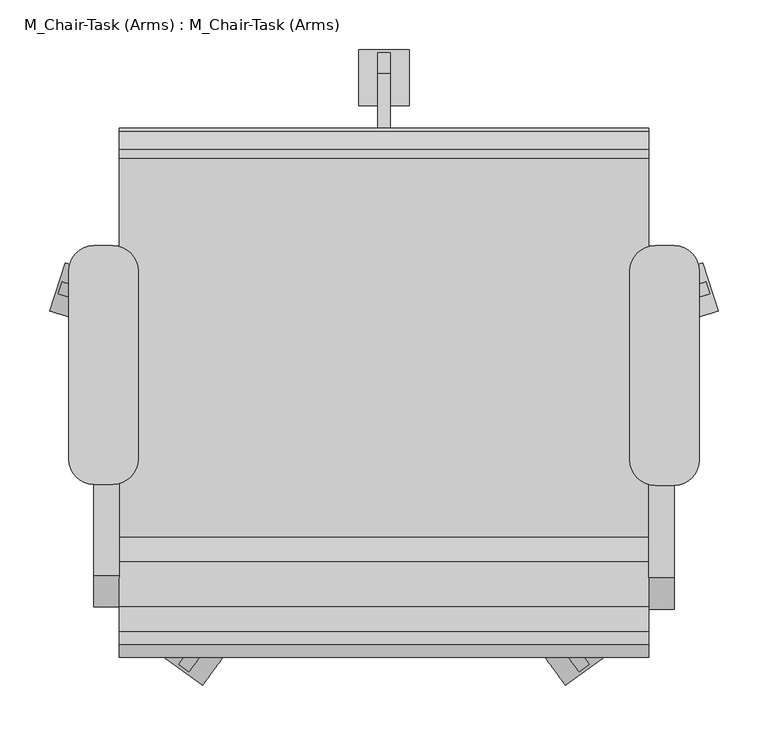
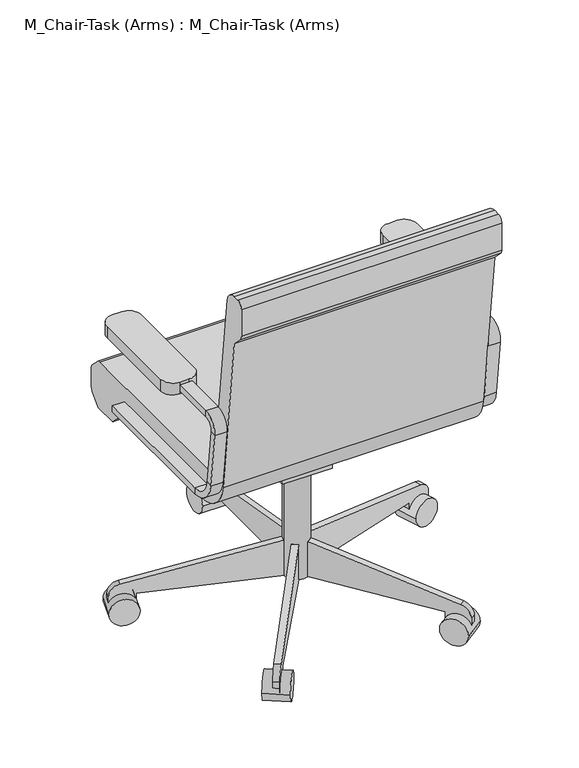
"""IFC4 building model written with IfcOpenShell, lengths in millimetres: furniture geometry, M_Chair-Task (Arms) : M_Chair-Task (Arms)."""

from ifc_helpers import new_model, si_unit, point, frame, frame_2d, origin, place, context, project, spatial, polyline, circle_curve, trimmed, segment, composite_curve, outline, extrude, source, transform, mapped, element, save
from ifc_brep_helpers import plane_surface, cylinder_surface, revolved_surface, advanced_brep


def m_chair_task_arms_m_chair_task_arms_bb362225(model_context):
    return source(origin(), model_context, "Body", "SolidModel", [
        extrude(outline(composite_curve([segment(polyline([(-126.2050455, 457.2), (255.0102301, 457.2)]), True, "CONTINUOUS"), segment(trimmed(circle_curve(frame_2d((255.0102301, 444.5)), 12.7), [point((255.0102301, 457.2))], [point((263.9604301, 453.510212))], False, "CARTESIAN"), True, "CONTINUOUS"), segment(polyline([(263.9604301, 453.510212), (281.8961016, 435.6939999)]), True, "CONTINUOUS"), segment(trimmed(circle_curve(frame_2d((272.9459016, 426.6837879)), 12.7), [point((281.8961016, 435.6939999))], [point((285.6459016, 426.6837879))], False, "CARTESIAN"), True, "CONTINUOUS"), segment(polyline([(285.6459016, 426.6837879), (285.6459016, 391.6405184)]), True, "CONTINUOUS"), segment(trimmed(circle_curve(frame_2d((260.2459016, 391.6405184)), 25.4), [point((285.6459016, 391.6405184))], [point((278.2663256, 373.7401184))], False, "CARTESIAN"), True, "CONTINUOUS"), segment(polyline([(278.2663256, 373.7401184), (260.2470284, 355.6), (209.4470284, 355.6), (181.0744602, 383.7835944), (-107.1089978, 383.7835944)]), True, "CONTINUOUS"), segment(trimmed(circle_curve(frame_2d((-107.1089978, 459.9835944)), 76.2), [point((-107.1089978, 383.7835944))], [point((-182.7870738, 451.0802913))], False, "CARTESIAN"), True, "CONTINUOUS"), segment(polyline([(-182.7870738, 451.0802913), (-222.3540984, 787.4), (-244.0343545, 809.0802561)]), True, "CONTINUOUS"), segment(trimmed(circle_curve(frame_2d((-235.0540984, 818.0605122)), 12.7), [point((-244.0343545, 809.0802561))], [point((-247.7540984, 818.0605122))], False, "CARTESIAN"), True, "CONTINUOUS"), segment(polyline([(-247.7540984, 818.0605122), (-247.7540984, 876.3)]), True, "CONTINUOUS"), segment(trimmed(circle_curve(frame_2d((-235.0540984, 876.3)), 12.7), [point((-247.7540984, 876.3))], [point((-235.0540984, 889.0))], False, "CARTESIAN"), True, "CONTINUOUS"), segment(polyline([(-235.0540984, 889.0), (-222.1789239, 889.0)]), True, "CONTINUOUS"), segment(trimmed(circle_curve(frame_2d((-222.1789239, 863.6)), 25.4), [point((-222.1789239, 889.0))], [point((-196.9528985, 866.5677677))], False, "CARTESIAN"), True, "CONTINUOUS"), segment(polyline([(-196.9528985, 866.5677677), (-151.4310708, 479.6322323)]), True, "CONTINUOUS"), segment(trimmed(circle_curve(frame_2d((-126.2050455, 482.6)), 25.4), [point((-151.4310708, 479.6322323))], [point((-126.2050455, 457.2))], True, "CARTESIAN"), True, "CONTINUOUS")], self_intersect=False)), frame((-125.7091803, 0.0, 0.0), z_axis=(1.0, 0.0, 0.0), x_axis=(0.0, 1.0, 0.0)), (0.0, 0.0, 1.0), 533.4),
        extrude(outline(polyline([(69.7459016, 383.7835944), (69.7459016, 371.0835944), (18.9459016, 283.0954134), (-19.1540984, 283.0954134), (-19.1540984, 383.7835944), (69.7459016, 383.7835944)])), frame((90.1908197, 0.0, 0.0), z_axis=(1.0, 0.0, 0.0), x_axis=(0.0, 1.0, 0.0)), (0.0, 0.0, 1.0), 101.6),
        extrude(outline(composite_curve([segment(polyline([(311.0459016, 53.5835944), (18.9459016, 53.5835944), (18.9459016, 129.7835944), (44.3459016, 129.7835944), (340.8565654, 77.5007643)]), True, "CONTINUOUS"), segment(trimmed(circle_curve(frame_2d((336.4459016, 52.4866474)), 25.4), [point((340.8565654, 77.5007643))], [point((361.8459016, 52.4866474))], False, "CARTESIAN"), True, "CONTINUOUS"), segment(polyline([(361.8459016, 52.4866474), (361.8459016, 28.1835944), (311.0459016, 28.1835944), (311.0459016, 53.5835944)]), True, "CONTINUOUS")], self_intersect=False)), frame((134.6408197, 0.0, 0.0), z_axis=(1.0, 0.0, 0.0), x_axis=(0.0, 1.0, 0.0)), (0.0, 0.0, 1.0), 12.7),
        extrude(outline(composite_curve([segment(trimmed(circle_curve(frame_2d((336.4459016, 28.1835944)), 28.2002727), [point((308.2456289, 28.1835944))], [point((364.6461744, 28.1835944))], False, "CARTESIAN"), True, "CONTINUOUS"), segment(trimmed(circle_curve(frame_2d((336.4459016, 28.1835944)), 28.2002727), [point((364.6461744, 28.1835944))], [point((308.2456289, 28.1835944))], False, "CARTESIAN"), True, "CONTINUOUS")], self_intersect=False)), frame((115.5908197, 0.0, 0.0), z_axis=(1.0, 0.0, 0.0), x_axis=(0.0, 1.0, 0.0)), (0.0, 0.0, 1.0), 50.8),
        extrude(outline(composite_curve([segment(polyline([(25.4, 0.0), (25.4, 292.1000001), (101.6, 292.1000001), (101.6, 266.7), (49.3171699, -29.8106636)]), True, "CONTINUOUS"), segment(trimmed(circle_curve(frame_2d((24.303053, -25.4)), 25.4), [point((49.3171699, -29.8106636))], [point((24.303053, -50.8))], False, "CARTESIAN"), True, "CONTINUOUS"), segment(polyline([(24.303053, -50.8), (0.0, -50.8), (0.0, 0.0), (25.4, 0.0)]), True, "CONTINUOUS")], self_intersect=False)), frame((-138.7750467, 103.1705568, 28.1835944), z_axis=(0.3090169943749487, 0.9510565162951532, 0.0), x_axis=(0.0, 0.0, 1.0)), (0.0, 0.0, 1.0), 12.7),
        extrude(outline(composite_curve([segment(trimmed(circle_curve(frame_2d((0.0, -28.2002727)), 28.2002727), [point((0.0, -56.4005454))], [point((0.0, 0.0))], False, "CARTESIAN"), True, "CONTINUOUS"), segment(trimmed(circle_curve(frame_2d((0.0, -28.2002727)), 28.2002727), [point((0.0, 0.0))], [point((0.0, -56.4005454))], False, "CARTESIAN"), True, "CONTINUOUS")], self_intersect=False)), frame((-195.638709, 101.6163254, 28.1835944), z_axis=(0.3090169943749487, 0.9510565162951532, 0.0), x_axis=(0.0, 0.0, -1.0)), (0.0, 0.0, 1.0), 50.8),
        extrude(outline(composite_curve([segment(polyline([(25.4, 0.0), (25.4, 292.1), (101.6, 292.1), (101.6, 266.7), (49.3171699, -29.8106637)]), True, "CONTINUOUS"), segment(trimmed(circle_curve(frame_2d((24.303053, -25.3999999)), 25.4), [point((49.3171699, -29.8106637))], [point((24.303053, -50.8))], False, "CARTESIAN"), True, "CONTINUOUS"), segment(polyline([(24.303053, -50.8), (0.0, -50.8), (0.0, 0.0), (25.4, 0.0)]), True, "CONTINUOUS")], self_intersect=False)), frame((-25.5639946, -221.1003988, 28.1835944), z_axis=(-0.8090169943749459, 0.5877852522924754, 0.0), x_axis=(0.0, 0.0, 1.0)), (0.0, 0.0, 1.0), 12.7),
        extrude(outline(composite_curve([segment(trimmed(circle_curve(frame_2d((0.0, -28.2002727)), 28.2002727), [point((0.0, -56.4005455))], [point((0.0, 0.0))], False, "CARTESIAN"), True, "CONTINUOUS"), segment(trimmed(circle_curve(frame_2d((0.0, -28.2002727)), 28.2002727), [point((0.0, 0.0))], [point((0.0, -56.4005455))], False, "CARTESIAN"), True, "CONTINUOUS")], self_intersect=False)), frame((-41.6576707, -275.6612394, 28.1835944), z_axis=(-0.8090169943749458, 0.5877852522924754, 0.0), x_axis=(0.0, 0.0, -1.0)), (0.0, 0.0, 1.0), 50.8),
        extrude(outline(composite_curve([segment(polyline([(-25.4, 0.0), (0.0, 0.0), (0.0, -50.8), (-24.303053, -50.8)]), True, "CONTINUOUS"), segment(trimmed(circle_curve(frame_2d((-24.303053, -25.3999999)), 25.4), [point((-24.303053, -50.8))], [point((-49.3171699, -29.8106636))], False, "CARTESIAN"), True, "CONTINUOUS"), segment(polyline([(-49.3171699, -29.8106636), (-101.6, 266.7), (-101.6, 292.1), (-25.4, 292.1), (-25.4, 0.0)]), True, "CONTINUOUS")], self_intersect=False)), frame((307.545634, -221.1003988, 28.1835944), z_axis=(0.8090169943749499, 0.5877852522924699, 0.0), x_axis=(0.0, 0.0, -1.0)), (0.0, 0.0, 1.0), 12.7),
        extrude(outline(composite_curve([segment(trimmed(circle_curve(frame_2d((0.0, -28.2002727)), 28.2002727), [point((0.0, -56.4005455))], [point((0.0, 0.0))], False, "CARTESIAN"), True, "CONTINUOUS"), segment(trimmed(circle_curve(frame_2d((0.0, -28.2002727)), 28.2002727), [point((0.0, 0.0))], [point((0.0, -56.4005455))], False, "CARTESIAN"), True, "CONTINUOUS")], self_intersect=False)), frame((323.63931, -275.6612394, 28.1835944), z_axis=(0.8090169943749499, 0.5877852522924699, 0.0), x_axis=(0.0, 0.0, 1.0)), (0.0, 0.0, 1.0), 50.8),
        extrude(outline(composite_curve([segment(polyline([(-25.4, 0.0), (0.0, 0.0), (0.0, -50.8), (-24.303053, -50.8)]), True, "CONTINUOUS"), segment(trimmed(circle_curve(frame_2d((-24.303053, -25.4)), 25.4), [point((-24.303053, -50.8))], [point((-49.3171699, -29.8106637))], False, "CARTESIAN"), True, "CONTINUOUS"), segment(polyline([(-49.3171699, -29.8106637), (-101.6, 266.7), (-101.6, 292.1), (-25.4, 292.1), (-25.4, 0.0)]), True, "CONTINUOUS")], self_intersect=False)), frame((420.756686, 103.1705568, 28.1835944), z_axis=(-0.3090169943749423, 0.9510565162951553, 0.0), x_axis=(0.0, 0.0, -1.0)), (0.0, 0.0, 1.0), 12.7),
        extrude(outline(composite_curve([segment(trimmed(circle_curve(frame_2d((0.0, -28.2002727)), 28.2002727), [point((0.0, -56.4005455))], [point((0.0, 0.0))], False, "CARTESIAN"), True, "CONTINUOUS"), segment(trimmed(circle_curve(frame_2d((0.0, -28.2002727)), 28.2002727), [point((0.0, 0.0))], [point((0.0, -56.4005455))], False, "CARTESIAN"), True, "CONTINUOUS")], self_intersect=False)), frame((477.6203484, 101.6163254, 28.1835944), z_axis=(-0.3090169943749423, 0.9510565162951553, 0.0), x_axis=(0.0, 0.0, 1.0)), (0.0, 0.0, 1.0), 50.8),
        extrude(outline(composite_curve([segment(trimmed(circle_curve(frame_2d((140.9908197, 18.9459016)), 25.4), [point((115.5908197, 18.9459016))], [point((166.3908197, 18.9459016))], False, "CARTESIAN"), True, "CONTINUOUS"), segment(trimmed(circle_curve(frame_2d((140.9908197, 18.9459016)), 25.4), [point((166.3908197, 18.9459016))], [point((115.5908197, 18.9459016))], False, "CARTESIAN"), True, "CONTINUOUS")], self_intersect=False)), frame((0.0, 0.0, 53.5835944), z_axis=(0.0, 0.0, 1.0), x_axis=(1.0, 0.0, 0.0)), (0.0, 0.0, 1.0), 330.5914056),
        advanced_brep(
        [(433.0908197, 167.0319091, 425.45), (433.0908197, 167.0319091, 412.75), (407.6908197, 167.0319091, 412.75), (407.6908197, 167.0319091, 425.45), (433.0908197, -128.329278, 425.45), (433.0908197, -128.329278, 412.75), (407.6908197, -128.329278, 412.75), (407.6908197, -128.329278, 425.45), (433.0908197, -185.0878351, 463.2225227), (433.0908197, -172.4748224, 464.7064065), (407.6908197, -185.0878351, 463.2225227), (407.6908197, -172.4748224, 464.7064065), (433.0908197, -186.2710303, 581.9741742), (433.0908197, -198.884043, 580.4902904), (407.6908197, -198.884043, 580.4902904), (407.6908197, -186.2710303, 581.9741742), (433.0908197, -167.3515113, 615.95), (433.0908197, -167.3515113, 603.25), (407.6908197, -167.3515113, 615.95), (407.6908197, -167.3515113, 603.25), (433.0908197, 18.9459016, 603.25), (407.6908197, 18.9459016, 603.25), (407.6908197, 18.9459016, 615.95), (433.0908197, 18.9459016, 615.95)],
        [
            (0, 1),
            (1, 2),
            (2, 3),
            (3, 0),
            (0, 4),
            (4, 5),
            (5, 1),
            (5, 6),
            (6, 2),
            (6, 7),
            (7, 3),
            (7, 4),
            (8, 5, circle_curve(frame((433.0908197, -128.329278, 469.9), z_axis=(1.0, 0.0, 0.0), x_axis=(0.0, 0.0, -1.0)), 57.15)),
            (4, 9, circle_curve(frame((433.0908197, -128.329278, 469.9), z_axis=(-1.0, 0.0, 0.0), x_axis=(0.0, 0.0, -1.0)), 44.45)),
            (9, 8),
            (10, 6, circle_curve(frame((407.6908197, -128.329278, 469.9), z_axis=(1.0, 0.0, 0.0), x_axis=(0.0, 0.0, -1.0)), 57.15)),
            (8, 10),
            (11, 7, circle_curve(frame((407.6908197, -128.329278, 469.9), z_axis=(1.0, 0.0, 0.0), x_axis=(0.0, 0.0, -1.0)), 44.45)),
            (10, 11),
            (11, 9),
            (9, 12),
            (12, 13),
            (13, 8),
            (13, 14),
            (14, 10),
            (14, 15),
            (15, 11),
            (15, 12),
            (16, 13, circle_curve(frame((433.0908197, -167.3515113, 584.2), z_axis=(1.0, 0.0, 0.0), x_axis=(0.0, -0.9931506043228767, -0.1168412475673929)), 31.75)),
            (12, 17, circle_curve(frame((433.0908197, -167.3515113, 584.2), z_axis=(-1.0, 0.0, 0.0), x_axis=(0.0, -0.9931506043228767, -0.1168412475673929)), 19.05)),
            (17, 16),
            (18, 14, circle_curve(frame((407.6908197, -167.3515113, 584.2), z_axis=(1.0, 0.0, 0.0), x_axis=(0.0, -0.9931506043228767, -0.1168412475673929)), 31.75)),
            (16, 18),
            (19, 15, circle_curve(frame((407.6908197, -167.3515113, 584.2), z_axis=(1.0, 0.0, 0.0), x_axis=(0.0, -0.9931506043228767, -0.1168412475673929)), 19.05)),
            (18, 19),
            (19, 17),
            (20, 21),
            (21, 22),
            (22, 23),
            (23, 20),
            (17, 20),
            (23, 16),
            (22, 18),
            (21, 19),
        ],
        [
            plane_surface(frame((406.191788, 167.0319091, 419.1), z_axis=(0.0, 1.0, 0.0), x_axis=(0.0, 0.0, -1.0))),
            plane_surface(frame((433.0908197, 167.0319091, 425.45), z_axis=(1.0, 0.0, 0.0), x_axis=(0.0, -1.0, 0.0))),
            plane_surface(frame((433.0908197, 167.0319091, 412.75), z_axis=(0.0, 0.0, -1.0), x_axis=(0.0, -1.0, 0.0))),
            plane_surface(frame((407.6908197, 167.0319091, 412.75), z_axis=(-1.0, 0.0, 0.0), x_axis=(0.0, -1.0, 0.0))),
            plane_surface(frame((407.6908197, 167.0319091, 425.45), z_axis=(0.0, 0.0, 1.0), x_axis=(0.0, -1.0, 0.0))),
            plane_surface(frame((433.0908197, -128.329278, 469.9), z_axis=(1.0, 0.0, 0.0), x_axis=(0.0, 0.0, -1.0))),
            cylinder_surface(frame((420.3908197, -128.329278, 469.9), z_axis=(-1.0, 0.0, 0.0), x_axis=(0.0, 0.0, -1.0)), 57.15),
            plane_surface(frame((407.6908197, -128.329278, 469.9), z_axis=(-1.0, 0.0, 0.0), x_axis=(0.0, 0.0, -1.0))),
            revolved_surface(polyline([(407.6908197, -128.329278, 425.45), (433.0908197, -128.329278, 425.45)]), (420.3908197, -128.329278, 469.9), (-1.0, 0.0, 0.0)),
            plane_surface(frame((433.0908197, -172.4748224, 464.7064065), z_axis=(1.0, 0.0, 0.0), x_axis=(0.0, -0.11684124756738626, 0.9931506043228775))),
            plane_surface(frame((433.0908197, -185.0878351, 463.2225227), z_axis=(0.0, -0.9931506043228775, -0.11684124756738655), x_axis=(0.0, -0.11684124756738655, 0.9931506043228775))),
            plane_surface(frame((407.6908197, -185.0878351, 463.2225227), z_axis=(-1.0, 0.0, 0.0), x_axis=(0.0, -0.11684124756738626, 0.9931506043228775))),
            plane_surface(frame((407.6908197, -172.4748224, 464.7064065), z_axis=(0.0, 0.9931506043228775, 0.11684124756738626), x_axis=(0.0, -0.11684124756738626, 0.9931506043228775))),
            plane_surface(frame((433.0908197, -167.3515113, 584.2), z_axis=(1.0, 0.0, 0.0), x_axis=(0.0, -0.9931506043228767, -0.1168412475673929))),
            cylinder_surface(frame((420.3908197, -167.3515113, 584.2), z_axis=(-1.0, 0.0, 0.0), x_axis=(0.0, -0.9931506043228767, -0.1168412475673929)), 31.75),
            plane_surface(frame((407.6908197, -167.3515113, 584.2), z_axis=(-1.0, 0.0, 0.0), x_axis=(0.0, -0.9931506043228767, -0.1168412475673929))),
            revolved_surface(polyline([(407.6908197, -186.2710303123508, 581.9741742338412), (433.0908197, -186.2710303123508, 581.9741742338412)]), (420.3908197, -167.3515113, 584.2), (-1.0, 0.0, 0.0)),
            plane_surface(frame((406.191788, 18.9459016, 609.6), z_axis=(0.0, 1.0, 0.0), x_axis=(0.0, 0.0, 1.0))),
            plane_surface(frame((433.0908197, -167.3515113, 603.25), z_axis=(1.0, 0.0, 0.0), x_axis=(0.0, 1.0, 0.0))),
            plane_surface(frame((433.0908197, -167.3515113, 615.95), z_axis=(0.0, 0.0, 1.0), x_axis=(0.0, 1.0, 0.0))),
            plane_surface(frame((407.6908197, -167.3515113, 615.95), z_axis=(-1.0, 0.0, 0.0), x_axis=(0.0, 1.0, 0.0))),
            plane_surface(frame((407.6908197, -167.3515113, 603.25), z_axis=(0.0, 0.0, -1.0), x_axis=(0.0, 1.0, 0.0))),
        ],
        [
            (0, [[1, 2, 3, 4]]),
            (1, [[-1, 5, 6, 7]]),
            (2, [[-2, -7, 8, 9]]),
            (3, [[-3, -9, 10, 11]]),
            (4, [[-4, -11, 12, -5]]),
            (5, [[13, -6, 14, 15]]),
            (6, [[16, -8, -13, 17]]),
            (7, [[18, -10, -16, 19]]),
            (8, [[-14, -12, -18, 20]]),
            (9, [[-15, 21, 22, 23]]),
            (10, [[-17, -23, 24, 25]]),
            (11, [[-19, -25, 26, 27]]),
            (12, [[-20, -27, 28, -21]]),
            (13, [[29, -22, 30, 31]]),
            (14, [[32, -24, -29, 33]]),
            (15, [[34, -26, -32, 35]]),
            (16, [[-30, -28, -34, 36]]),
            (17, [[37, 38, 39, 40]]),
            (18, [[-31, 41, -40, 42]]),
            (19, [[-33, -42, -39, 43]]),
            (20, [[-35, -43, -38, 44]]),
            (21, [[-36, -44, -37, -41]]),
        ],
    ),
        advanced_brep(
        [(-151.1091803, 167.0319091, 412.75), (-151.1091803, 167.0319091, 425.45), (-125.7091803, 167.0319091, 425.45), (-125.7091803, 167.0319091, 412.75), (-151.1091803, -126.2388651, 412.75), (-151.1091803, -126.2388651, 425.45), (-125.7091803, -126.2388651, 425.45), (-125.7091803, -126.2388651, 412.75), (-151.1091803, -170.3844094, 464.7064065), (-151.1091803, -182.9974221, 463.2225227), (-125.7091803, -170.3844094, 464.7064065), (-125.7091803, -182.9974221, 463.2225227), (-151.1091803, -196.7936301, 580.4902904), (-151.1091803, -184.1806174, 581.9741742), (-125.7091803, -184.1806174, 581.9741742), (-125.7091803, -196.7936301, 580.4902904), (-151.1091803, -165.2610984, 603.25), (-151.1091803, -165.2610984, 615.95), (-125.7091803, -165.2610984, 603.25), (-125.7091803, -165.2610984, 615.95), (-151.1091803, 18.9459016, 615.95), (-125.7091803, 18.9459016, 615.95), (-125.7091803, 18.9459016, 603.25), (-151.1091803, 18.9459016, 603.25)],
        [
            (0, 1),
            (1, 2),
            (2, 3),
            (3, 0),
            (0, 4),
            (4, 5),
            (5, 1),
            (5, 6),
            (6, 2),
            (6, 7),
            (7, 3),
            (7, 4),
            (8, 5, circle_curve(frame((-151.1091803, -126.2388651, 469.9), z_axis=(1.0, 0.0, 0.0), x_axis=(0.0, 0.0, -1.0)), 44.45)),
            (4, 9, circle_curve(frame((-151.1091803, -126.2388651, 469.9), z_axis=(-1.0, 0.0, 0.0), x_axis=(0.0, 0.0, -1.0)), 57.15)),
            (9, 8),
            (10, 6, circle_curve(frame((-125.7091803, -126.2388651, 469.9), z_axis=(1.0, 0.0, 0.0), x_axis=(0.0, 0.0, -1.0)), 44.45)),
            (8, 10),
            (11, 7, circle_curve(frame((-125.7091803, -126.2388651, 469.9), z_axis=(1.0, 0.0, 0.0), x_axis=(0.0, 0.0, -1.0)), 57.15)),
            (10, 11),
            (11, 9),
            (9, 12),
            (12, 13),
            (13, 8),
            (13, 14),
            (14, 10),
            (14, 15),
            (15, 11),
            (15, 12),
            (16, 13, circle_curve(frame((-151.1091803, -165.2610984, 584.2), z_axis=(1.0, 0.0, 0.0), x_axis=(0.0, -0.9931506043228768, -0.11684124756739202)), 19.05)),
            (12, 17, circle_curve(frame((-151.1091803, -165.2610984, 584.2), z_axis=(-1.0, 0.0, 0.0), x_axis=(0.0, -0.9931506043228768, -0.11684124756739202)), 31.75)),
            (17, 16),
            (18, 14, circle_curve(frame((-125.7091803, -165.2610984, 584.2), z_axis=(1.0, 0.0, 0.0), x_axis=(0.0, -0.9931506043228768, -0.11684124756739202)), 19.05)),
            (16, 18),
            (19, 15, circle_curve(frame((-125.7091803, -165.2610984, 584.2), z_axis=(1.0, 0.0, 0.0), x_axis=(0.0, -0.9931506043228768, -0.11684124756739202)), 31.75)),
            (18, 19),
            (19, 17),
            (20, 21),
            (21, 22),
            (22, 23),
            (23, 20),
            (17, 20),
            (23, 16),
            (22, 18),
            (21, 19),
        ],
        [
            plane_surface(frame((-152.608212, 167.0319091, 419.1), z_axis=(0.0, 1.0, 0.0), x_axis=(0.0, 0.0, -1.0))),
            plane_surface(frame((-151.1091803, 167.0319091, 412.75), z_axis=(-1.0, 0.0, 0.0), x_axis=(0.0, -1.0, 0.0))),
            plane_surface(frame((-151.1091803, 167.0319091, 425.45), z_axis=(0.0, 0.0, 1.0), x_axis=(0.0, -1.0, 0.0))),
            plane_surface(frame((-125.7091803, 167.0319091, 425.45), z_axis=(1.0, 0.0, 0.0), x_axis=(0.0, -1.0, 0.0))),
            plane_surface(frame((-125.7091803, 167.0319091, 412.75), z_axis=(0.0, 0.0, -1.0), x_axis=(0.0, -1.0, 0.0))),
            plane_surface(frame((-151.1091803, -126.2388651, 469.9), z_axis=(-1.0, 0.0, 0.0), x_axis=(0.0, 0.0, -1.0))),
            revolved_surface(polyline([(-151.1091803, -126.2388651, 425.45), (-125.7091803, -126.2388651, 425.45)]), (-138.4091803, -126.2388651, 469.9), (-1.0, 0.0, 0.0)),
            plane_surface(frame((-125.7091803, -126.2388651, 469.9), z_axis=(1.0, 0.0, 0.0), x_axis=(0.0, 0.0, -1.0))),
            cylinder_surface(frame((-138.4091803, -126.2388651, 469.9), z_axis=(-1.0, 0.0, 0.0), x_axis=(0.0, 0.0, -1.0)), 57.15),
            plane_surface(frame((-151.1091803, -182.9974221, 463.2225227), z_axis=(-1.0, 0.0, 0.0), x_axis=(0.0, -0.1168412475673856, 0.9931506043228776))),
            plane_surface(frame((-151.1091803, -170.3844094, 464.7064065), z_axis=(0.0, 0.9931506043228776, 0.1168412475673856), x_axis=(0.0, -0.1168412475673856, 0.9931506043228776))),
            plane_surface(frame((-125.7091803, -170.3844094, 464.7064065), z_axis=(1.0, 0.0, 0.0), x_axis=(0.0, -0.1168412475673856, 0.9931506043228776))),
            plane_surface(frame((-125.7091803, -182.9974221, 463.2225227), z_axis=(0.0, -0.9931506043228776, -0.1168412475673856), x_axis=(0.0, -0.1168412475673856, 0.9931506043228776))),
            plane_surface(frame((-151.1091803, -165.2610984, 584.2), z_axis=(-1.0, 0.0, 0.0), x_axis=(0.0, -0.9931506043228768, -0.11684124756739202))),
            revolved_surface(polyline([(-151.1091803, -184.1806174123508, 581.9741742338413), (-125.7091803, -184.1806174123508, 581.9741742338413)]), (-138.4091803, -165.2610984, 584.2), (-1.0, 0.0, 0.0)),
            plane_surface(frame((-125.7091803, -165.2610984, 584.2), z_axis=(1.0, 0.0, 0.0), x_axis=(0.0, -0.9931506043228768, -0.11684124756739202))),
            cylinder_surface(frame((-138.4091803, -165.2610984, 584.2), z_axis=(-1.0, 0.0, 0.0), x_axis=(0.0, -0.9931506043228768, -0.11684124756739202)), 31.75),
            plane_surface(frame((-152.608212, 18.9459016, 609.6), z_axis=(0.0, 1.0, 0.0), x_axis=(0.0, 0.0, 1.0))),
            plane_surface(frame((-151.1091803, -165.2610984, 615.95), z_axis=(-1.0, 0.0, 0.0), x_axis=(0.0, 1.0, 0.0))),
            plane_surface(frame((-151.1091803, -165.2610984, 603.25), z_axis=(0.0, 0.0, -1.0), x_axis=(0.0, 1.0, 0.0))),
            plane_surface(frame((-125.7091803, -165.2610984, 603.25), z_axis=(1.0, 0.0, 0.0), x_axis=(0.0, 1.0, 0.0))),
            plane_surface(frame((-125.7091803, -165.2610984, 615.95), z_axis=(0.0, 0.0, 1.0), x_axis=(0.0, 1.0, 0.0))),
        ],
        [
            (0, [[1, 2, 3, 4]]),
            (1, [[-1, 5, 6, 7]]),
            (2, [[-2, -7, 8, 9]]),
            (3, [[-3, -9, 10, 11]]),
            (4, [[-4, -11, 12, -5]]),
            (5, [[13, -6, 14, 15]]),
            (6, [[16, -8, -13, 17]]),
            (7, [[18, -10, -16, 19]]),
            (8, [[-14, -12, -18, 20]]),
            (9, [[-15, 21, 22, 23]]),
            (10, [[-17, -23, 24, 25]]),
            (11, [[-19, -25, 26, 27]]),
            (12, [[-20, -27, 28, -21]]),
            (13, [[29, -22, 30, 31]]),
            (14, [[32, -24, -29, 33]]),
            (15, [[34, -26, -32, 35]]),
            (16, [[-30, -28, -34, 36]]),
            (17, [[37, 38, 39, 40]]),
            (18, [[-31, 41, -40, 42]]),
            (19, [[-33, -42, -39, 43]]),
            (20, [[-35, -43, -38, 44]]),
            (21, [[-36, -44, -37, -41]]),
        ],
    ),
        extrude(outline(composite_curve([segment(polyline([(433.0908197, -74.2028048), (414.0408197, -74.2028048)]), True, "CONTINUOUS"), segment(trimmed(circle_curve(frame_2d((414.0408197, -48.8028048)), 25.4), [point((414.0408197, -74.2028048))], [point((388.6408197, -48.8028048))], False, "CARTESIAN"), True, "CONTINUOUS"), segment(polyline([(388.6408197, -48.8028048), (388.6408197, 141.6319091)]), True, "CONTINUOUS"), segment(trimmed(circle_curve(frame_2d((414.0408197, 141.6319091)), 25.4), [point((388.6408197, 141.6319091))], [point((414.0408197, 167.0319091))], False, "CARTESIAN"), True, "CONTINUOUS"), segment(polyline([(414.0408197, 167.0319091), (433.0908197, 167.0319091)]), True, "CONTINUOUS"), segment(trimmed(circle_curve(frame_2d((433.0908197, 141.6319091)), 25.4), [point((433.0908197, 167.0319091))], [point((458.4908197, 141.6319091))], False, "CARTESIAN"), True, "CONTINUOUS"), segment(polyline([(458.4908197, 141.6319091), (458.4908197, -48.8028048)]), True, "CONTINUOUS"), segment(trimmed(circle_curve(frame_2d((433.0908197, -48.8028048)), 25.4), [point((458.4908197, -48.8028048))], [point((433.0908197, -74.2028048))], False, "CARTESIAN"), True, "CONTINUOUS")], self_intersect=False)), frame((0.0, 0.0, 596.9), z_axis=(0.0, 0.0, 1.0), x_axis=(1.0, 0.0, 0.0)), (0.0, 0.0, 1.0), 25.4),
        extrude(outline(composite_curve([segment(polyline([(-132.0591803, -73.1575984), (-151.1091803, -73.1575984)]), True, "CONTINUOUS"), segment(trimmed(circle_curve(frame_2d((-151.1091803, -47.7575984)), 25.4), [point((-151.1091803, -73.1575984))], [point((-176.5091803, -47.7575984))], False, "CARTESIAN"), True, "CONTINUOUS"), segment(polyline([(-176.5091803, -47.7575984), (-176.5091803, 141.6319091)]), True, "CONTINUOUS"), segment(trimmed(circle_curve(frame_2d((-151.1091803, 141.6319091)), 25.4), [point((-176.5091803, 141.6319091))], [point((-151.1091803, 167.0319091))], False, "CARTESIAN"), True, "CONTINUOUS"), segment(polyline([(-151.1091803, 167.0319091), (-132.0591803, 167.0319091)]), True, "CONTINUOUS"), segment(trimmed(circle_curve(frame_2d((-132.0591803, 141.6319091)), 25.4), [point((-132.0591803, 167.0319091))], [point((-106.6591803, 141.6319091))], False, "CARTESIAN"), True, "CONTINUOUS"), segment(polyline([(-106.6591803, 141.6319091), (-106.6591803, -47.7575984)]), True, "CONTINUOUS"), segment(trimmed(circle_curve(frame_2d((-132.0591803, -47.7575984)), 25.4), [point((-106.6591803, -47.7575984))], [point((-132.0591803, -73.1575984))], False, "CARTESIAN"), True, "CONTINUOUS")], self_intersect=False)), frame((0.0, 0.0, 596.9), z_axis=(0.0, 0.0, 1.0), x_axis=(1.0, 0.0, 0.0)), (0.0, 0.0, 1.0), 25.4),
    ])


if __name__ == "__main__":
    model = new_model("IFC4")
    model_context = context("Model", 3, world=origin())
    ifc_project = project(units=[si_unit("LENGTHUNIT", "METRE", prefix="MILLI")], contexts=[model_context])
    site = spatial("IfcSite", under=ifc_project)
    building = spatial("IfcBuilding", under=site)
    placement = place(None, origin())
    m_chair_task_arms_m_chair_task_arms_shape = m_chair_task_arms_m_chair_task_arms_bb362225(model_context)
    element("IfcFurniture", 1, ObjectType="M_Chair-Task (Arms) : M_Chair-Task (Arms)", at=placement, inside=building, context=model_context, shape_type="MappedRepresentation", body=[
        mapped(m_chair_task_arms_m_chair_task_arms_shape, transform((0.0, 0.0, 0.0), x_axis=(1.0, 0.0, 0.0), y_axis=(0.0, 1.0, 0.0), z_axis=(0.0, 0.0, 1.0))),
    ])
    save(model, "model.ifc")

# Revit data of these elements
# Type "M_Chair-Task (Arms) : M_Chair-Task (Arms)"
#   Base Material = Plastic, Opaque Black
#   Caster Material = Plastic, Opaque Black
#   Seat/Back Material = Textile - Slate Blue
#   Default Elevation = 0
# Element 1 (IfcFurniture, "M_Chair-Task (Arms) : M_Chair-Task (Arms)")
#   Materials on its faces: "Plastic, Opaque Black", "Textile - Slate Blue"
# Materials
#   "Plastic, Opaque Black": class "Plastic", colour RGB 0 0 0, transparency 0.7, Description = "Plastic, generic, opaque black", Cost = 0
#   "Textile - Slate Blue": class "Fabric", colour RGB 98 102 118, transparency 0
